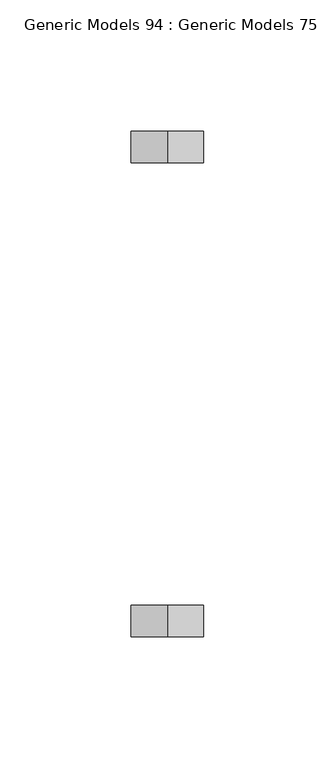
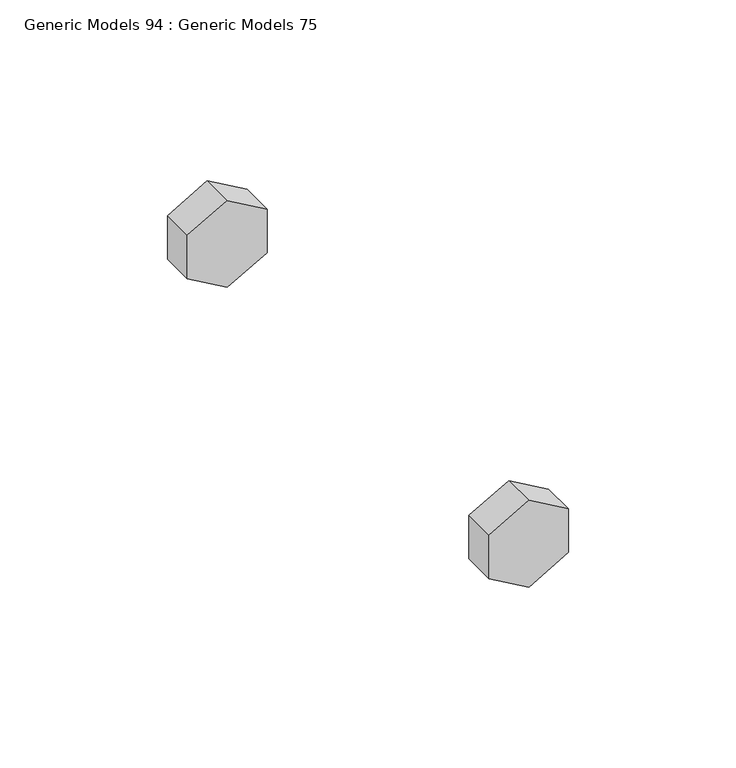
"""IFC4 building model written with IfcOpenShell, lengths in millimetres: proxy geometry, Generic Models 94 : Generic Models 75."""

from ifc_helpers import new_model, si_unit, frame, origin, place, context, project, spatial, polyline, outline, extrude, source, transform, mapped, element, save


def generic_models_94_generic_models_75_9a4f5ebf(model_context):
    return source(origin(), model_context, "Body", "SweptSolid", [
        extrude(outline(polyline([(268536.8902933, 31974.4067029), (268521.0537198, 31974.4067029), (268513.135433, 31988.1215778), (268521.0537198, 32001.8364528), (268536.8902933, 32001.8364528), (268544.80858, 31988.1215778), (268536.8902933, 31974.4067029)])), frame((0.0, 36491.5582942, 0.0), z_axis=(0.0, 1.0, 0.0), x_axis=(0.0, 0.0, 1.0)), (0.0, 0.0, 1.0), 11.90625),
        extrude(outline(polyline([(268536.8902933, 31974.4067029), (268521.0537198, 31974.4067029), (268513.135433, 31988.1215778), (268521.0537198, 32001.8364528), (268536.8902933, 32001.8364528), (268544.80858, 31988.1215778), (268536.8902933, 31974.4067029)])), frame((0.0, 36311.3770442, 0.0), z_axis=(0.0, 1.0, 0.0), x_axis=(0.0, 0.0, 1.0)), (0.0, 0.0, 1.0), 11.90625),
    ])


if __name__ == "__main__":
    model = new_model("IFC4")
    model_context = context("Model", 3, world=origin())
    ifc_project = project(units=[si_unit("LENGTHUNIT", "METRE", prefix="MILLI")], contexts=[model_context])
    site = spatial("IfcSite", under=ifc_project)
    building = spatial("IfcBuilding", under=site)
    placement = place(None, origin())
    generic_models_94_generic_models_75_shape = generic_models_94_generic_models_75_9a4f5ebf(model_context)
    element("IfcBuildingElementProxy", 1, Name="Generic Models 94 : Generic Models 75", ObjectType="Generic Models 94 : Generic Models 75", at=placement, inside=building, context=model_context, shape_type="MappedRepresentation", body=[
        mapped(generic_models_94_generic_models_75_shape, transform((0.0, 0.0, 0.0), x_axis=(1.0, 0.0, 0.0), y_axis=(0.0, 1.0, 0.0), z_axis=(0.0, 0.0, 1.0))),
    ])
    save(model, "model.ifc")

# Revit data of these elements
# Element 1 (IfcBuildingElementProxy, "Generic Models 94 : Generic Models 75")
#   Materials on its faces: "3/4\" GALV. THRU BOLTS"
# Materials
#   "3/4\" GALV. THRU BOLTS": class "Generic", colour RGB 105 69 171, transparency 0, Cost = 0
